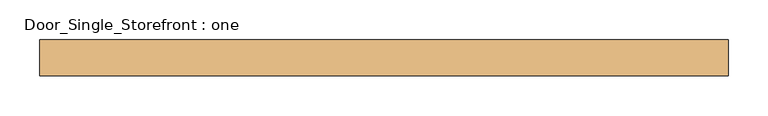
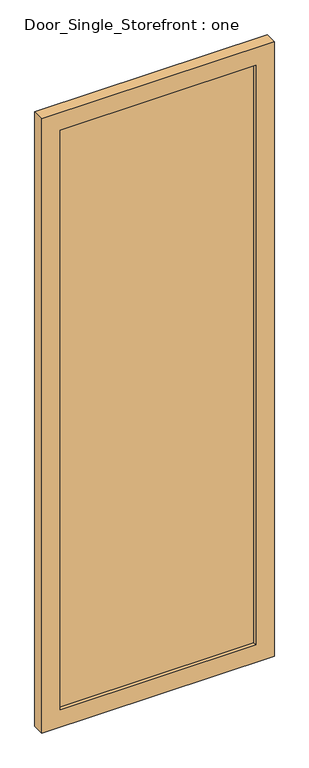
"""IFC4 building model written with IfcOpenShell, lengths in millimetres: door geometry, Door_Single_Storefront : one."""

from ifc_helpers import new_model, si_unit, frame, origin, place, context, project, spatial, polyline, outline, extrude, source, transform, mapped, element, save


def door_single_storefront_one_ca385b29(model_context):
    return source(origin(), model_context, "Body", "SweptSolid", [
        extrude(outline(polyline([(361.766159, -6.35), (-361.766159, -6.35), (-361.766159, 12.7), (361.766159, 12.7), (361.766159, -6.35)])), frame((0.0, 0.0, 68.2625), z_axis=(0.0, 0.0, 1.0), x_axis=(1.0, 0.0, 0.0)), (0.0, 0.0, 1.0), 2263.3107725),
        extrude(outline(polyline([(2399.8357725, -430.028659), (0.0, -430.028659), (0.0, 430.028659), (2399.8357725, 430.028659), (2399.8357725, -430.028659)]), holes=[polyline([(68.2625, 361.766159), (68.2625, -361.766159), (2331.5732725, -361.766159), (2331.5732725, 361.766159), (68.2625, 361.766159)])]), frame((0.0, -19.05, 0.0), z_axis=(0.0, 1.0, 0.0), x_axis=(0.0, 0.0, 1.0)), (0.0, 0.0, 1.0), 44.45),
    ])


if __name__ == "__main__":
    model = new_model("IFC4")
    model_context = context("Model", 3, world=origin())
    ifc_project = project(units=[si_unit("LENGTHUNIT", "METRE", prefix="MILLI")], contexts=[model_context])
    site = spatial("IfcSite", under=ifc_project)
    building = spatial("IfcBuilding", under=site)
    placement = place(None, origin())
    door_single_storefront_one_shape = door_single_storefront_one_ca385b29(model_context)
    element("IfcDoor", 1, ObjectType="Door_Single_Storefront : one", at=placement, inside=building, context=model_context, shape_type="MappedRepresentation", body=[
        mapped(door_single_storefront_one_shape, transform((0.0, 0.0, 0.0), x_axis=(1.0, 0.0, 0.0), y_axis=(0.0, 1.0, 0.0), z_axis=(0.0, 0.0, 1.0))),
    ])
    save(model, "model.ifc")

# Revit data of these elements
# Type "Door_Single_Storefront : one"
#   Type Mark = "29"
#   OD_DS_Door_Material = "ALUM./GLAZING"
#   OD_DS_Door_Type = "STOREFRONT (NARROW STILE)"
#   OD_DS_Lockset = "ENTRY LOCK (INSIDE ADA LEVER ALWAYS ACTIVE)"
#   Analytic Construction = "<None>"
#   angle open [instance default] = 132.952°
#   Stile_Width = 0' - 2 11/16"
#   Door_Thickness = 0' - 1 3/4"
#   Door_Offset = 0' - 1"
#   Glass_Material = TEMPERED INSULATED GLAZING (CARDINAL GLASS LoĒ²-240\nOR EQUIVALENT)
#   Frame_Material = KAWNEER 260 INSULCLADTM THERMAL ENTRANCE - CLEAR ANODIZED ALUM.
#   Function = (empty or 0)
# Element 1 (IfcDoor, "Door_Single_Storefront : one")
#   angle open = 90.00°
#   Materials on its faces: "KAWNEER 260 INSULCLADTM THERMAL ENTRANCE - CLEAR ANODIZED ALUM.", "TEMPERED INSULATED GLAZING (CARDINAL GLASS LoĒ²-240\nOR EQUIVALENT)"
# Materials
#   "TEMPERED INSULATED GLAZING (CARDINAL GLASS LoĒ²-240\nOR EQUIVALENT)": class "Glass", colour RGB 196 205 210, transparency 0.85, Description = "Soda Lime Glass", Cost = 0
#   "KAWNEER 260 INSULCLADTM THERMAL ENTRANCE - CLEAR ANODIZED ALUM.": class "Metal", colour RGB 244 244 244, transparency 0, Description = "Aluminum 6061", Cost = 0
